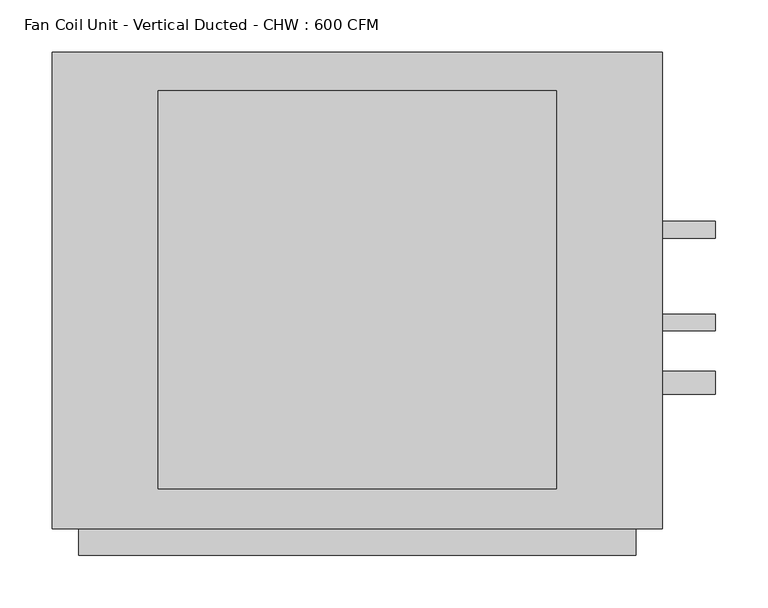
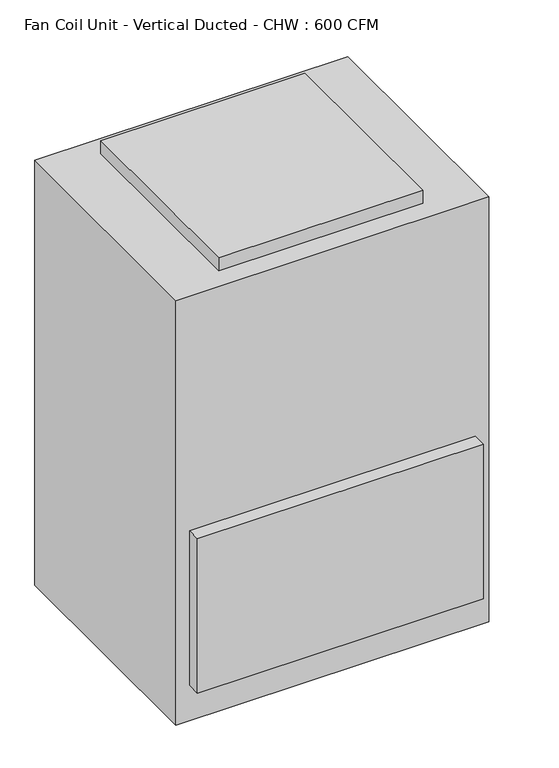
"""IFC4 building model written with IfcOpenShell, lengths in millimetres: proxy geometry, Fan Coil Unit - Vertical Ducted - CHW : 600 CFM."""

import ifcopenshell
import ifcopenshell.guid

model = None  # the IFC model being written
_history = None  # IfcOwnerHistory: only IFC2X3 demands one
_inside = {}  # id of a spatial element -> (the spatial element, [elements in it])
_under = {}  # id of a project, library or spatial element -> (it, [spatial elements below it])
_declared = {}  # id of a project -> (the project, [libraries it declares])
_typed = {}  # id of a type object -> (the type object, [elements of that type])
_made_of = {}  # id of a material, layer set ... -> (it, [elements and type objects made of it])


def new_model(schema):
    """Start an empty IFC model of exactly this schema.

    Asked for "IFC4X3", IfcOpenShell would pick the latest addendum, in which some entities
    have other attributes; the version numbers below select the first issue.
    IFC2X3 requires an IfcOwnerHistory on every rooted entity: one is made here for all.
    """
    global model, _history
    if schema == "IFC4X3":
        model = ifcopenshell.file(schema_version=(4, 3, 0, 0))
    else:
        model = ifcopenshell.file(schema=schema)
    _inside.clear()
    _under.clear()
    _declared.clear()
    _typed.clear()
    _made_of.clear()
    _history = None
    if model.schema == "IFC2X3":
        org = make("IfcOrganization", Name="unknown")
        user = make(
            "IfcPersonAndOrganization",
            ThePerson=make("IfcPerson", FamilyName="unknown"),
            TheOrganization=org,
        )
        app = make(
            "IfcApplication",
            ApplicationDeveloper=org,
            Version="unknown",
            ApplicationFullName="unknown",
            ApplicationIdentifier="unknown",
        )
        _history = make(
            "IfcOwnerHistory",
            OwningUser=user,
            OwningApplication=app,
            ChangeAction="ADDED",
            CreationDate=0,
        )
    return model


def make(cls, **values):
    """One entity of the class cls with the attributes given. An attribute that is None is left unset."""
    return model.create_entity(
        cls, **{name: value for name, value in values.items() if value is not None}
    )


def rooted(cls, **values):
    """An entity with a GlobalId (a new one), such as an element, a storey or a relation."""
    return make(cls, GlobalId=ifcopenshell.guid.new(), OwnerHistory=_history, **values)


def si_unit(unit_type, name, prefix=None):
    """IfcSIUnit, for example si_unit("LENGTHUNIT", "METRE", prefix="MILLI")."""
    return make("IfcSIUnit", UnitType=unit_type, Prefix=prefix, Name=name)


def assignment(units):
    """IfcUnitAssignment: the units of a project."""
    return None if units is None else make("IfcUnitAssignment", Units=units)


def point(xyz):
    """IfcCartesianPoint."""
    return None if xyz is None else make("IfcCartesianPoint", Coordinates=xyz)


def direction(xyz):
    """IfcDirection."""
    return None if xyz is None else make("IfcDirection", DirectionRatios=xyz)


def frame(location, z_axis=None, x_axis=None):
    """IfcAxis2Placement3D, a coordinate frame: its origin and axes. An axis left out is left unset."""
    return make(
        "IfcAxis2Placement3D",
        Location=point(location),
        Axis=direction(z_axis),
        RefDirection=direction(x_axis),
    )


def origin():
    """The frame at (0, 0, 0) with its axes left unset."""
    return frame((0.0, 0.0, 0.0))


def place(relative_to, where):
    """IfcLocalPlacement: puts the frame where relative to a parent placement (None: the world)."""
    return make(
        "IfcLocalPlacement", PlacementRelTo=relative_to, RelativePlacement=where
    )


def context(
    kind, dimensions, precision=None, world=None, true_north=None, identifier=None
):
    """IfcGeometricRepresentationContext, for example the 3D "Model" context."""
    return make(
        "IfcGeometricRepresentationContext",
        ContextIdentifier=identifier,
        ContextType=kind,
        CoordinateSpaceDimension=dimensions,
        Precision=precision,
        WorldCoordinateSystem=world,
        TrueNorth=true_north,
    )


def project(units=None, contexts=None):
    """IfcProject with its units and contexts."""
    return rooted(
        "IfcProject",
        Name="project",
        RepresentationContexts=contexts,
        UnitsInContext=assignment(units),
    )


def spatial(cls, under=None, at=None, **own):
    """A site, building, storey or space (cls), placed at a placement, below another one or the project."""
    s = rooted(cls, ObjectPlacement=at, **own)
    if under is not None:
        _under.setdefault(under.id(), (under, []))[1].append(s)
    return s


def circle_curve(where, radius):
    """IfcCircle in the frame where."""
    return make("IfcCircle", Position=where, Radius=radius)


def shape(context_of_items, identifier, shape_type, items):
    """IfcShapeRepresentation: the items that make up one representation, for example the "Body"."""
    return make(
        "IfcShapeRepresentation",
        ContextOfItems=context_of_items,
        RepresentationIdentifier=identifier,
        RepresentationType=shape_type,
        Items=items,
    )


def source(mapping_origin, context_of_items, identifier, shape_type, items):
    """IfcRepresentationMap: a shape defined once, which mapped items show again and again."""
    return make(
        "IfcRepresentationMap",
        MappingOrigin=mapping_origin,
        MappedRepresentation=shape(context_of_items, identifier, shape_type, items),
    )


def transform(
    local_origin,
    x_axis=None,
    y_axis=None,
    z_axis=None,
    scale=None,
    scale2=None,
    scale3=None,
    uniform=True,
):
    """IfcCartesianTransformationOperator3D, or its non-uniform kind. x_axis, y_axis, z_axis: its Axis1, 2, 3."""
    if uniform:
        return make(
            "IfcCartesianTransformationOperator3D",
            Axis1=direction(x_axis),
            Axis2=direction(y_axis),
            LocalOrigin=point(local_origin),
            Scale=scale,
            Axis3=direction(z_axis),
        )
    return make(
        "IfcCartesianTransformationOperator3DnonUniform",
        Axis1=direction(x_axis),
        Axis2=direction(y_axis),
        LocalOrigin=point(local_origin),
        Scale=scale,
        Axis3=direction(z_axis),
        Scale2=scale2,
        Scale3=scale3,
    )


def mapped(mapping_source, mapping_target):
    """IfcMappedItem: shows the shape of a source again, moved by a transform."""
    return make(
        "IfcMappedItem", MappingSource=mapping_source, MappingTarget=mapping_target
    )


def made_of(thing, what):
    """Note that an element or type object is made of a material, layer set ...; save() writes the relation."""
    if what is not None:
        _made_of.setdefault(what.id(), (what, []))[1].append(thing)
    return thing


def element(
    cls,
    number,
    at=None,
    inside=None,
    cuts=None,
    type_object=None,
    material=None,
    context=None,
    identifier="Body",
    shape_type=None,
    held_by="IfcProductDefinitionShape",
    body=None,
    shapes=None,
    **own,
):
    """One element of the class cls, such as IfcWall. Its Tag is "e" and its number.

    at: its placement. inside: the storey or other place that contains it. cuts: it is an
    opening in that element (IfcRelVoidsElement). A single representation is given by context,
    identifier, shape_type and body (its items); several are given by shapes. held_by: the class
    of the entity that holds the representations. save() writes the other relations.
    """
    e = rooted(cls, Tag="e%d" % number, ObjectPlacement=at, **own)
    if body is not None:
        shapes = [shape(context, identifier, shape_type, body)]
    if shapes is not None:
        e.Representation = make(held_by, Representations=shapes)
    if inside is not None:
        _inside.setdefault(inside.id(), (inside, []))[1].append(e)
    if cuts is not None:
        rooted(
            "IfcRelVoidsElement", RelatingBuildingElement=cuts, RelatedOpeningElement=e
        )
    if type_object is not None:
        _typed.setdefault(type_object.id(), (type_object, []))[1].append(e)
    return made_of(e, material)


def aggregate(whole, parts):
    """IfcRelAggregates: a whole, such as a stair, and the parts it consists of."""
    return rooted("IfcRelAggregates", RelatingObject=whole, RelatedObjects=parts)


def save(model, path):
    """Write the relations noted so far, then the file.

    IfcRelAggregates (storeys below a building ...), IfcRelContainedInSpatialStructure (elements
    in a storey), IfcRelDefinesByType, IfcRelAssociatesMaterial and IfcRelDeclares: one each for
    every whole, place, type object, material and project.
    """
    for whole, parts in _under.values():
        aggregate(whole, parts)
    for where, things in _inside.values():
        rooted(
            "IfcRelContainedInSpatialStructure",
            RelatedElements=things,
            RelatingStructure=where,
        )
    for kind, things in _typed.values():
        rooted("IfcRelDefinesByType", RelatedObjects=things, RelatingType=kind)
    for what, things in _made_of.values():
        rooted("IfcRelAssociatesMaterial", RelatedObjects=things, RelatingMaterial=what)
    for by, libraries in _declared.values():
        rooted("IfcRelDeclares", RelatingContext=by, RelatedDefinitions=libraries)
    model.write(path)


def plane_surface(at):
    """IfcPlane: the flat surface through the origin of the frame at, square to its z axis."""
    return make("IfcPlane", Position=at)


def cylinder_surface(at, radius):
    """IfcCylindricalSurface: all points at the distance radius from the z axis of the frame at."""
    return make("IfcCylindricalSurface", Position=at, Radius=radius)


def advanced_brep(points, edges, surfaces, faces):
    """IfcAdvancedBrep: a solid bounded by faces that lie on surfaces and meet in shared edges.

    An edge is (start, end): straight between two places in points (the first is 0);
    or (start, end, curve); or (start, end, curve, False) where it runs against its curve.
    A face is (place in surfaces, loops), or (place, loops, False) where it looks against
    its surface's normal. A loop lists edges by number (the first is 1), with a minus sign
    where the edge is run from its end to its start. The first loop is the outer one.
    """
    corners = [point(p) for p in points]
    vertices = [make("IfcVertexPoint", VertexGeometry=c) for c in corners]
    made = []
    for start, end, *more in edges:
        made.append(
            make(
                "IfcEdgeCurve",
                EdgeStart=vertices[start],
                EdgeEnd=vertices[end],
                EdgeGeometry=more[0] if more else make("IfcPolyline", Points=[corners[start], corners[end]]),
                SameSense=more[1] if len(more) > 1 else True,
            )
        )
    hull = []
    for where, loops, *sense in faces:
        bounds = []
        for j, loop in enumerate(loops):
            ring = [make("IfcOrientedEdge", EdgeElement=made[abs(k) - 1], Orientation=k > 0) for k in loop]
            bounds.append(
                make(
                    "IfcFaceOuterBound" if j == 0 else "IfcFaceBound",
                    Bound=make("IfcEdgeLoop", EdgeList=ring),
                    Orientation=True,
                )
            )
        hull.append(make("IfcAdvancedFace", Bounds=bounds, FaceSurface=surfaces[where], SameSense=sense[0] if sense else True))
    return make("IfcAdvancedBrep", Outer=make("IfcClosedShell", CfsFaces=hull))


def fan_coil_unit_vertical_ducted_chw_600_cfm_7dbe3da6(model_context):
    return source(origin(), model_context, "Body", "AdvancedBrep", [
        advanced_brep(
        [(482.6, 419.1, 863.6), (101.6, 419.1, 863.6), (101.6, 38.1, 863.6), (482.6, 38.1, 863.6), (482.6, 419.1, 838.2), (101.6, 419.1, 838.2), (101.6, 38.1, 838.2), (482.6, 38.1, 838.2), (584.2, 455.901774, 838.2), (0.0, 455.901774, 838.2), (0.0, 0.0, 838.2), (584.2, 0.0, 838.2), (584.2, 455.901774, 0.0), (584.2, 0.0, 0.0), (0.0, 0.0, 0.0), (0.0, 455.901774, 0.0), (25.4, 0.0, 374.65), (558.8, 0.0, 374.65), (558.8, 0.0, 69.85), (25.4, 0.0, 69.85), (584.2, 293.976774, 673.1), (584.2, 278.101774, 673.1), (584.2, 205.076774, 593.725), (584.2, 189.201774, 593.725), (584.2, 150.8125, 431.8), (584.2, 128.5875, 431.8), (558.8, -25.4, 374.65), (25.4, -25.4, 374.65), (25.4, -25.4, 69.85), (558.8, -25.4, 69.85), (635.0, 278.101774, 673.1), (635.0, 293.976774, 673.1), (635.0, 189.201774, 593.725), (635.0, 205.076774, 593.725), (635.0, 128.5875, 431.8), (635.0, 150.8125, 431.8)],
        [
            (0, 1),
            (1, 2),
            (2, 3),
            (3, 0),
            (0, 4),
            (4, 5),
            (5, 1),
            (5, 6),
            (6, 2),
            (6, 7),
            (7, 3),
            (7, 4),
            (8, 9),
            (9, 10),
            (10, 11),
            (11, 8),
            (12, 13),
            (13, 14),
            (14, 15),
            (15, 12),
            (8, 12),
            (15, 9),
            (14, 10),
            (13, 11),
            (16, 17),
            (17, 18),
            (18, 19),
            (19, 16),
            (20, 21, circle_curve(frame((584.2, 286.039274, 673.1), z_axis=(-1.0, 0.0, 0.0), x_axis=(0.0, 1.0, 0.0)), 7.9375)),
            (21, 20, circle_curve(frame((584.2, 286.039274, 673.1), z_axis=(-1.0, 0.0, 0.0), x_axis=(0.0, 1.0, 0.0)), 7.9375)),
            (22, 23, circle_curve(frame((584.2, 197.139274, 593.725), z_axis=(-1.0, 0.0, 0.0), x_axis=(0.0, 1.0, 0.0)), 7.9375)),
            (23, 22, circle_curve(frame((584.2, 197.139274, 593.725), z_axis=(-1.0, 0.0, 0.0), x_axis=(0.0, 1.0, 0.0)), 7.9375)),
            (24, 25, circle_curve(frame((584.2, 139.7, 431.8), z_axis=(-1.0, 0.0, 0.0), x_axis=(0.0, 1.0, 0.0)), 11.1125)),
            (25, 24, circle_curve(frame((584.2, 139.7, 431.8), z_axis=(-1.0, 0.0, 0.0), x_axis=(0.0, 1.0, 0.0)), 11.1125)),
            (26, 27),
            (27, 28),
            (28, 29),
            (29, 26),
            (26, 17),
            (16, 27),
            (19, 28),
            (18, 29),
            (30, 31, circle_curve(frame((635.0, 286.039274, 673.1), z_axis=(1.0, 0.0, 0.0), x_axis=(0.0, 1.0, 0.0)), 7.9375)),
            (31, 30, circle_curve(frame((635.0, 286.039274, 673.1), z_axis=(1.0, 0.0, 0.0), x_axis=(0.0, 1.0, 0.0)), 7.9375)),
            (30, 21),
            (20, 31),
            (32, 33, circle_curve(frame((635.0, 197.139274, 593.725), z_axis=(1.0, 0.0, 0.0), x_axis=(0.0, 1.0, 0.0)), 7.9375)),
            (33, 32, circle_curve(frame((635.0, 197.139274, 593.725), z_axis=(1.0, 0.0, 0.0), x_axis=(0.0, 1.0, 0.0)), 7.9375)),
            (32, 23),
            (22, 33),
            (34, 35, circle_curve(frame((635.0, 139.7, 431.8), z_axis=(1.0, 0.0, 0.0), x_axis=(0.0, 1.0, 0.0)), 11.1125)),
            (35, 34, circle_curve(frame((635.0, 139.7, 431.8), z_axis=(1.0, 0.0, 0.0), x_axis=(0.0, 1.0, 0.0)), 11.1125)),
            (34, 25),
            (24, 35),
        ],
        [
            plane_surface(frame((101.6, 419.1, 863.6), z_axis=(0.0, 0.0, 1.0), x_axis=(-1.0, 0.0, 0.0))),
            plane_surface(frame((482.6, 419.1, 863.6), z_axis=(0.0, 1.0, 0.0), x_axis=(0.0, 0.0, -1.0))),
            plane_surface(frame((101.6, 419.1, 863.6), z_axis=(-1.0, 0.0, 0.0), x_axis=(0.0, 0.0, -1.0))),
            plane_surface(frame((101.6, 38.1, 863.6), z_axis=(0.0, -1.0, 0.0), x_axis=(0.0, 0.0, -1.0))),
            plane_surface(frame((482.6, 38.1, 863.6), z_axis=(1.0, 0.0, 0.0), x_axis=(0.0, 0.0, -1.0))),
            plane_surface(frame((0.0, 455.901774, 838.2), z_axis=(0.0, 0.0, 1.0), x_axis=(-1.0, 0.0, 0.0))),
            plane_surface(frame((0.0, 455.901774, 0.0), z_axis=(0.0, 0.0, -1.0), x_axis=(1.0, 0.0, 0.0))),
            plane_surface(frame((584.2, 455.901774, 838.2), z_axis=(0.0, 1.0, 0.0), x_axis=(0.0, 0.0, -1.0))),
            plane_surface(frame((0.0, 455.901774, 838.2), z_axis=(-1.0, 0.0, 0.0), x_axis=(0.0, 0.0, -1.0))),
            plane_surface(frame((0.0, 0.0, 838.2), z_axis=(0.0, -1.0, 0.0), x_axis=(0.0, 0.0, -1.0))),
            plane_surface(frame((584.2, 0.0, 838.2), z_axis=(1.0, 0.0, 0.0), x_axis=(0.0, 0.0, -1.0))),
            plane_surface(frame((25.4, -25.4, 374.65), z_axis=(0.0, -1.0, 0.0), x_axis=(-1.0, 0.0, 0.0))),
            plane_surface(frame((558.8, -25.4, 374.65), z_axis=(0.0, 0.0, 1.0), x_axis=(0.0, 1.0, 0.0))),
            plane_surface(frame((25.4, -25.4, 374.65), z_axis=(-1.0, 0.0, 0.0), x_axis=(0.0, 1.0, 0.0))),
            plane_surface(frame((25.4, -25.4, 69.85), z_axis=(0.0, 0.0, -1.0), x_axis=(0.0, 1.0, 0.0))),
            plane_surface(frame((558.8, -25.4, 69.85), z_axis=(1.0, 0.0, 0.0), x_axis=(0.0, 1.0, 0.0))),
            plane_surface(frame((635.0, 293.976774, 673.1), z_axis=(1.0, 0.0, 0.0), x_axis=(0.0, 0.0, 1.0))),
            cylinder_surface(frame((584.2, 286.039274, 673.1), z_axis=(1.0, 0.0, 0.0), x_axis=(0.0, 1.0, 0.0)), 7.9375),
            plane_surface(frame((635.0, 205.076774, 593.725), z_axis=(1.0, 0.0, 0.0), x_axis=(0.0, 0.0, 1.0))),
            cylinder_surface(frame((584.2, 197.139274, 593.725), z_axis=(1.0, 0.0, 0.0), x_axis=(0.0, 1.0, 0.0)), 7.9375),
            plane_surface(frame((635.0, 150.8125, 431.8), z_axis=(1.0, 0.0, 0.0), x_axis=(0.0, 0.0, 1.0))),
            cylinder_surface(frame((584.2, 139.7, 431.8), z_axis=(1.0, 0.0, 0.0), x_axis=(0.0, 1.0, 0.0)), 11.1125),
        ],
        [
            (0, [[1, 2, 3, 4]]),
            (1, [[-1, 5, 6, 7]]),
            (2, [[-2, -7, 8, 9]]),
            (3, [[-3, -9, 10, 11]]),
            (4, [[-4, -11, 12, -5]]),
            (5, [[13, 14, 15, 16], [-6, -12, -10, -8]]),
            (6, [[17, 18, 19, 20]]),
            (7, [[-13, 21, -20, 22]]),
            (8, [[-14, -22, -19, 23]]),
            (9, [[-15, -23, -18, 24], [25, 26, 27, 28]]),
            (10, [[-16, -24, -17, -21], [29, 30], [31, 32], [33, 34]]),
            (11, [[35, 36, 37, 38]]),
            (12, [[-35, 39, -25, 40]]),
            (13, [[-36, -40, -28, 41]]),
            (14, [[-37, -41, -27, 42]]),
            (15, [[-38, -42, -26, -39]]),
            (16, [[43, 44]]),
            (17, [[-43, 45, -29, 46]]),
            (17, [[-44, -46, -30, -45]]),
            (18, [[47, 48]]),
            (19, [[-47, 49, -31, 50]]),
            (19, [[-48, -50, -32, -49]]),
            (20, [[51, 52]]),
            (21, [[-51, 53, -33, 54]]),
            (21, [[-52, -54, -34, -53]]),
        ],
    ),
    ])


if __name__ == "__main__":
    model = new_model("IFC4")
    model_context = context("Model", 3, world=origin())
    ifc_project = project(units=[si_unit("LENGTHUNIT", "METRE", prefix="MILLI")], contexts=[model_context])
    site = spatial("IfcSite", under=ifc_project)
    building = spatial("IfcBuilding", under=site)
    placement = place(None, origin())
    fan_coil_unit_vertical_ducted_chw_600_cfm_shape = fan_coil_unit_vertical_ducted_chw_600_cfm_7dbe3da6(model_context)
    element("IfcBuildingElementProxy", 1, Name="Fan Coil Unit - Vertical Ducted - CHW : 600 CFM", ObjectType="Fan Coil Unit - Vertical Ducted - CHW : 600 CFM", at=placement, inside=building, context=model_context, shape_type="MappedRepresentation", body=[
        mapped(fan_coil_unit_vertical_ducted_chw_600_cfm_shape, transform((0.0, 0.0, 0.0), x_axis=(1.0, 0.0, 0.0), y_axis=(0.0, 1.0, 0.0), z_axis=(0.0, 0.0, 1.0))),
    ])
    save(model, "model.ifc")

# Revit data of these elements
# Type "Fan Coil Unit - Vertical Ducted - CHW : 600 CFM"
#   COBie.Type.CreatedBy = "design@eagle.com"
#   COBie.Type.CreatedOn = "2016-10-27T05:31:12"
#   COBie.Type.Name = "Fan Coil Unit - Vertical Ducted - CHW_600 CFM"
#   COBie.Type.Category = "23-75 70 17 27 : Fan Coil Units"
#   COBie.Type.Description = "Fan Coil Unit - Vertical Ducted - CHW_600 CFM"
#   COBie.Type.Manufacturer = ""
#   COBie.Type.ModelNumber = ""
#   COBie.Type.ReplacementCost = 0
#   Water Pressure Drop [instance default] = 1.40 psi
#   Voltage = 240 V
#   Unit Length = 1' - 11"
#   Total Cooling Capacity = 19700 Btu/h
#   Supply Air Width = 15"
#   Sensible Cooling Capacity = 14400 Btu/h
#   Return Air Width = 21"
#   Nominal Air Flow [instance default] = 600 CFM
#   External Static Pressure [instance default] = 0.30 in-wg
#   Drain Flow [instance default] = 0 GPM
#   Chilled Water Flow [instance default] = 4 GPM
#   C2 Offset 1 = 0' - 6 11/16"
#   Apparent Load = 265 VA
#   COBie.Type = yes
#   Number of Poles = 2
#   Load Classification = Cooling
#   CFU Material = none
